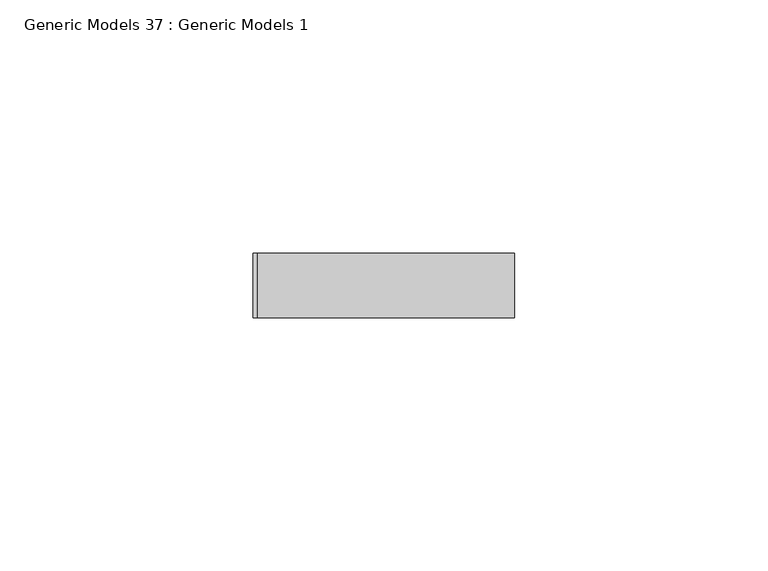
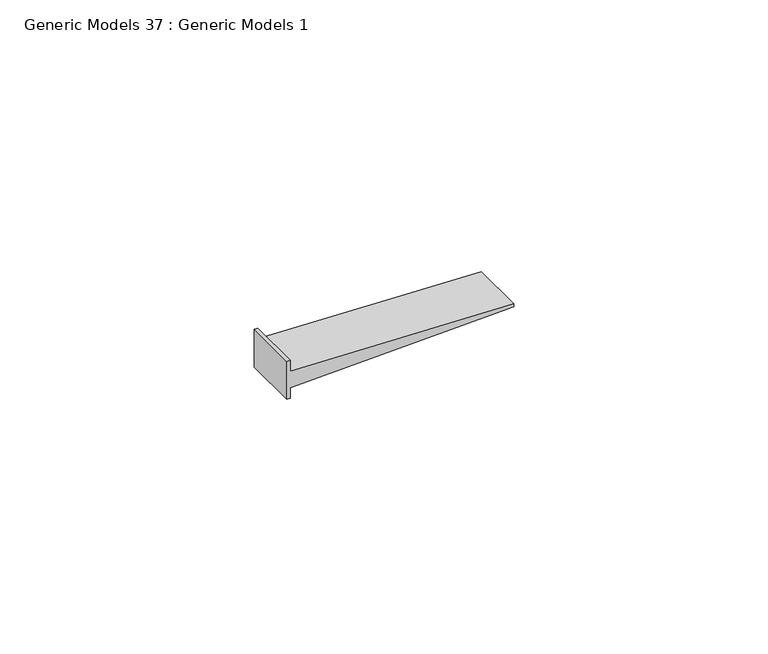
"""IFC4 building model written with IfcOpenShell, lengths in millimetres: proxy geometry, Generic Models 37 : Generic Models 1."""

import ifcopenshell
import ifcopenshell.guid

model = None  # the IFC model being written
_history = None  # IfcOwnerHistory: only IFC2X3 demands one
_inside = {}  # id of a spatial element -> (the spatial element, [elements in it])
_under = {}  # id of a project, library or spatial element -> (it, [spatial elements below it])
_declared = {}  # id of a project -> (the project, [libraries it declares])
_typed = {}  # id of a type object -> (the type object, [elements of that type])
_made_of = {}  # id of a material, layer set ... -> (it, [elements and type objects made of it])


def new_model(schema):
    """Start an empty IFC model of exactly this schema.

    Asked for "IFC4X3", IfcOpenShell would pick the latest addendum, in which some entities
    have other attributes; the version numbers below select the first issue.
    IFC2X3 requires an IfcOwnerHistory on every rooted entity: one is made here for all.
    """
    global model, _history
    if schema == "IFC4X3":
        model = ifcopenshell.file(schema_version=(4, 3, 0, 0))
    else:
        model = ifcopenshell.file(schema=schema)
    _inside.clear()
    _under.clear()
    _declared.clear()
    _typed.clear()
    _made_of.clear()
    _history = None
    if model.schema == "IFC2X3":
        org = make("IfcOrganization", Name="unknown")
        user = make(
            "IfcPersonAndOrganization",
            ThePerson=make("IfcPerson", FamilyName="unknown"),
            TheOrganization=org,
        )
        app = make(
            "IfcApplication",
            ApplicationDeveloper=org,
            Version="unknown",
            ApplicationFullName="unknown",
            ApplicationIdentifier="unknown",
        )
        _history = make(
            "IfcOwnerHistory",
            OwningUser=user,
            OwningApplication=app,
            ChangeAction="ADDED",
            CreationDate=0,
        )
    return model


def make(cls, **values):
    """One entity of the class cls with the attributes given. An attribute that is None is left unset."""
    return model.create_entity(
        cls, **{name: value for name, value in values.items() if value is not None}
    )


def rooted(cls, **values):
    """An entity with a GlobalId (a new one), such as an element, a storey or a relation."""
    return make(cls, GlobalId=ifcopenshell.guid.new(), OwnerHistory=_history, **values)


def si_unit(unit_type, name, prefix=None):
    """IfcSIUnit, for example si_unit("LENGTHUNIT", "METRE", prefix="MILLI")."""
    return make("IfcSIUnit", UnitType=unit_type, Prefix=prefix, Name=name)


def assignment(units):
    """IfcUnitAssignment: the units of a project."""
    return None if units is None else make("IfcUnitAssignment", Units=units)


def point(xyz):
    """IfcCartesianPoint."""
    return None if xyz is None else make("IfcCartesianPoint", Coordinates=xyz)


def direction(xyz):
    """IfcDirection."""
    return None if xyz is None else make("IfcDirection", DirectionRatios=xyz)


def frame(location, z_axis=None, x_axis=None):
    """IfcAxis2Placement3D, a coordinate frame: its origin and axes. An axis left out is left unset."""
    return make(
        "IfcAxis2Placement3D",
        Location=point(location),
        Axis=direction(z_axis),
        RefDirection=direction(x_axis),
    )


def origin():
    """The frame at (0, 0, 0) with its axes left unset."""
    return frame((0.0, 0.0, 0.0))


def place(relative_to, where):
    """IfcLocalPlacement: puts the frame where relative to a parent placement (None: the world)."""
    return make(
        "IfcLocalPlacement", PlacementRelTo=relative_to, RelativePlacement=where
    )


def context(
    kind, dimensions, precision=None, world=None, true_north=None, identifier=None
):
    """IfcGeometricRepresentationContext, for example the 3D "Model" context."""
    return make(
        "IfcGeometricRepresentationContext",
        ContextIdentifier=identifier,
        ContextType=kind,
        CoordinateSpaceDimension=dimensions,
        Precision=precision,
        WorldCoordinateSystem=world,
        TrueNorth=true_north,
    )


def project(units=None, contexts=None):
    """IfcProject with its units and contexts."""
    return rooted(
        "IfcProject",
        Name="project",
        RepresentationContexts=contexts,
        UnitsInContext=assignment(units),
    )


def spatial(cls, under=None, at=None, **own):
    """A site, building, storey or space (cls), placed at a placement, below another one or the project."""
    s = rooted(cls, ObjectPlacement=at, **own)
    if under is not None:
        _under.setdefault(under.id(), (under, []))[1].append(s)
    return s


def polyline(points):
    """IfcPolyline through the points."""
    return make("IfcPolyline", Points=[point(p) for p in points])


def outline(outer, holes=None, kind="AREA"):
    """IfcArbitraryClosedProfileDef: a profile drawn as a closed curve; with holes, ...WithVoids."""
    if holes is None:
        return make("IfcArbitraryClosedProfileDef", ProfileType=kind, OuterCurve=outer)
    return make(
        "IfcArbitraryProfileDefWithVoids",
        ProfileType=kind,
        OuterCurve=outer,
        InnerCurves=holes,
    )


def extrude(swept, where, along, depth):
    """IfcExtrudedAreaSolid: the profile swept, set in the frame where, extruded along a direction by depth."""
    return make(
        "IfcExtrudedAreaSolid",
        SweptArea=swept,
        Position=where,
        ExtrudedDirection=direction(along),
        Depth=depth,
    )


def shape(context_of_items, identifier, shape_type, items):
    """IfcShapeRepresentation: the items that make up one representation, for example the "Body"."""
    return make(
        "IfcShapeRepresentation",
        ContextOfItems=context_of_items,
        RepresentationIdentifier=identifier,
        RepresentationType=shape_type,
        Items=items,
    )


def source(mapping_origin, context_of_items, identifier, shape_type, items):
    """IfcRepresentationMap: a shape defined once, which mapped items show again and again."""
    return make(
        "IfcRepresentationMap",
        MappingOrigin=mapping_origin,
        MappedRepresentation=shape(context_of_items, identifier, shape_type, items),
    )


def transform(
    local_origin,
    x_axis=None,
    y_axis=None,
    z_axis=None,
    scale=None,
    scale2=None,
    scale3=None,
    uniform=True,
):
    """IfcCartesianTransformationOperator3D, or its non-uniform kind. x_axis, y_axis, z_axis: its Axis1, 2, 3."""
    if uniform:
        return make(
            "IfcCartesianTransformationOperator3D",
            Axis1=direction(x_axis),
            Axis2=direction(y_axis),
            LocalOrigin=point(local_origin),
            Scale=scale,
            Axis3=direction(z_axis),
        )
    return make(
        "IfcCartesianTransformationOperator3DnonUniform",
        Axis1=direction(x_axis),
        Axis2=direction(y_axis),
        LocalOrigin=point(local_origin),
        Scale=scale,
        Axis3=direction(z_axis),
        Scale2=scale2,
        Scale3=scale3,
    )


def mapped(mapping_source, mapping_target):
    """IfcMappedItem: shows the shape of a source again, moved by a transform."""
    return make(
        "IfcMappedItem", MappingSource=mapping_source, MappingTarget=mapping_target
    )


def made_of(thing, what):
    """Note that an element or type object is made of a material, layer set ...; save() writes the relation."""
    if what is not None:
        _made_of.setdefault(what.id(), (what, []))[1].append(thing)
    return thing


def element(
    cls,
    number,
    at=None,
    inside=None,
    cuts=None,
    type_object=None,
    material=None,
    context=None,
    identifier="Body",
    shape_type=None,
    held_by="IfcProductDefinitionShape",
    body=None,
    shapes=None,
    **own,
):
    """One element of the class cls, such as IfcWall. Its Tag is "e" and its number.

    at: its placement. inside: the storey or other place that contains it. cuts: it is an
    opening in that element (IfcRelVoidsElement). A single representation is given by context,
    identifier, shape_type and body (its items); several are given by shapes. held_by: the class
    of the entity that holds the representations. save() writes the other relations.
    """
    e = rooted(cls, Tag="e%d" % number, ObjectPlacement=at, **own)
    if body is not None:
        shapes = [shape(context, identifier, shape_type, body)]
    if shapes is not None:
        e.Representation = make(held_by, Representations=shapes)
    if inside is not None:
        _inside.setdefault(inside.id(), (inside, []))[1].append(e)
    if cuts is not None:
        rooted(
            "IfcRelVoidsElement", RelatingBuildingElement=cuts, RelatedOpeningElement=e
        )
    if type_object is not None:
        _typed.setdefault(type_object.id(), (type_object, []))[1].append(e)
    return made_of(e, material)


def aggregate(whole, parts):
    """IfcRelAggregates: a whole, such as a stair, and the parts it consists of."""
    return rooted("IfcRelAggregates", RelatingObject=whole, RelatedObjects=parts)


def save(model, path):
    """Write the relations noted so far, then the file.

    IfcRelAggregates (storeys below a building ...), IfcRelContainedInSpatialStructure (elements
    in a storey), IfcRelDefinesByType, IfcRelAssociatesMaterial and IfcRelDeclares: one each for
    every whole, place, type object, material and project.
    """
    for whole, parts in _under.values():
        aggregate(whole, parts)
    for where, things in _inside.values():
        rooted(
            "IfcRelContainedInSpatialStructure",
            RelatedElements=things,
            RelatingStructure=where,
        )
    for kind, things in _typed.values():
        rooted("IfcRelDefinesByType", RelatedObjects=things, RelatingType=kind)
    for what, things in _made_of.values():
        rooted("IfcRelAssociatesMaterial", RelatedObjects=things, RelatingMaterial=what)
    for by, libraries in _declared.values():
        rooted("IfcRelDeclares", RelatingContext=by, RelatedDefinitions=libraries)
    model.write(path)


def generic_models_37_generic_models_1_d2f23889(model_context):
    return source(origin(), model_context, "Body", "SweptSolid", [
        extrude(outline(polyline([(485.1617794, 52541.7008608), (476.0685794, 52541.7008608), (476.0685794, 52542.4946108), (478.618443, 52542.4946108), (480.2158321, 52593.2946108), (481.0145267, 52593.2946108), (482.6119158, 52542.4946108), (485.1617794, 52542.4946108), (485.1617794, 52541.7008608)])), frame((0.0, 565.15, 0.0), z_axis=(0.0, 1.0, 0.0), x_axis=(0.0, 0.0, 1.0)), (0.0, 0.0, 1.0), 12.7),
    ])


if __name__ == "__main__":
    model = new_model("IFC4")
    model_context = context("Model", 3, world=origin())
    ifc_project = project(units=[si_unit("LENGTHUNIT", "METRE", prefix="MILLI")], contexts=[model_context])
    site = spatial("IfcSite", under=ifc_project)
    building = spatial("IfcBuilding", under=site)
    placement = place(None, origin())
    generic_models_37_generic_models_1_shape = generic_models_37_generic_models_1_d2f23889(model_context)
    element("IfcBuildingElementProxy", 1, Name="Generic Models 37 : Generic Models 1", ObjectType="Generic Models 37 : Generic Models 1", at=placement, inside=building, context=model_context, shape_type="MappedRepresentation", body=[
        mapped(generic_models_37_generic_models_1_shape, transform((0.0, 0.0, 0.0), x_axis=(1.0, 0.0, 0.0), y_axis=(0.0, 1.0, 0.0), z_axis=(0.0, 0.0, 1.0))),
    ])
    save(model, "model.ifc")

# Revit data of these elements
# Element 1 (IfcBuildingElementProxy, "Generic Models 37 : Generic Models 1")
#   Materials on its faces: "ATTACH GYPSUM BOARD TO STUDS AND NOT TO TOP TRACK"
# Materials
#   "ATTACH GYPSUM BOARD TO STUDS AND NOT TO TOP TRACK": class "Generic", colour RGB 48 48 48, transparency 0, Cost = 0
